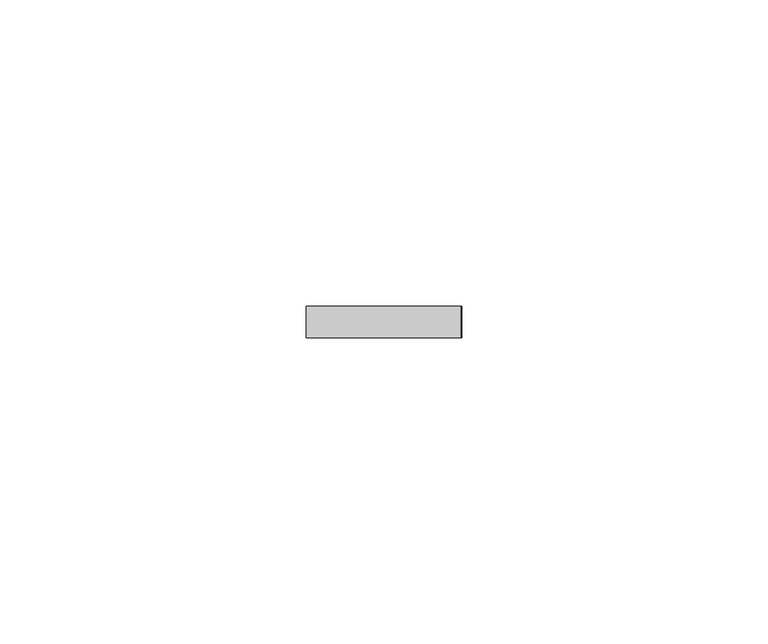
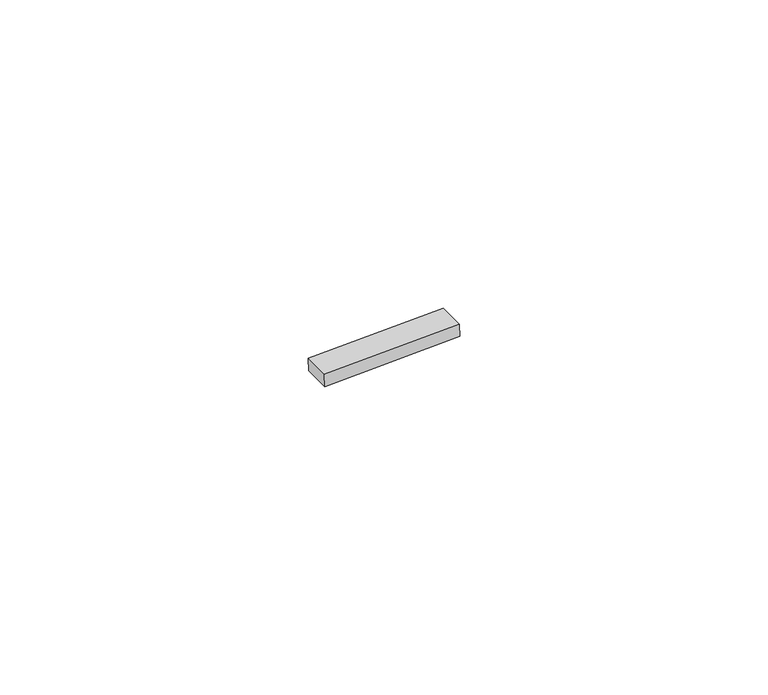
"""IFC4 building model written with IfcOpenShell, lengths in millimetres: proxy geometry, Inner panel:Inner panel:1:Inner panel:1 : Inner panel:Inner panel:300324:2:Inner panel:1:Inner panel:1 : Inner panel:Inner panel:300324:2 : Inner panel:Inner panel:1:Inner panel:1 : Inner panel:Inner panel:300324:300043:149 : Inner panel:Inner panel:1:Inner panel:1 : Inner panel:Inner panel:300324:2:Inner panel:1:Inner panel:1 : Inner panel:Inner panel:300324:2 : Inner panel:Inner panel:1:Inner panel:1 : Inner panel:Inner panel:300324:300043:308120."""

from ifc_helpers import new_model, si_unit, frame, origin, place, context, project, spatial, polyline, outline, extrude, source, transform, mapped, element, save


def generic_models_3277445f(model_context):
    return source(origin(), model_context, "Body", "SweptSolid", [
        extrude(outline(polyline([(0.0, -25.3999999), (0.0, 0.0), (5.2138089, 0.0), (5.2138089, -25.3999999), (0.0, -25.3999999)])), frame((558296.2989334, -578534.9848948, 3863.6749017), z_axis=(-0.041630544712223896, 0.0, 0.9991330730923502), x_axis=(0.0, -1.0, 0.0)), (0.0, 0.0, 1.0), 2.4763745),
    ])


if __name__ == "__main__":
    model = new_model("IFC4")
    model_context = context("Model", 3, world=origin())
    ifc_project = project(units=[si_unit("LENGTHUNIT", "METRE", prefix="MILLI")], contexts=[model_context])
    site = spatial("IfcSite", under=ifc_project)
    building = spatial("IfcBuilding", under=site)
    placement = place(None, origin())
    generic_models_shape = generic_models_3277445f(model_context)
    element("IfcBuildingElementProxy", 1, Name="Inner panel:Inner panel:1:Inner panel:1 : Inner panel:Inner panel:300324:2:Inner panel:1:Inner panel:1 : Inner panel:Inner panel:300324:2 : Inner panel:Inner panel:1:Inner panel:1 : Inner panel:Inner panel:300324:300043:149 : Inner panel:Inner panel:1:Inner panel:1 : Inner panel:Inner panel:300324:2:Inner panel:1:Inner panel:1 : Inner panel:Inner panel:300324:2 : Inner panel:Inner panel:1:Inner panel:1 : Inner panel:Inner panel:300324:300043:308120", ObjectType="Inner panel:Inner panel:1:Inner panel:1 : Inner panel:Inner panel:300324:2:Inner panel:1:Inner panel:1 : Inner panel:Inner panel:300324:2 : Inner panel:Inner panel:1:Inner panel:1 : Inner panel:Inner panel:300324:300043:149 : Inner panel:Inner panel:1:Inner panel:1 : Inner panel:Inner panel:300324:2:Inner panel:1:Inner panel:1 : Inner panel:Inner panel:300324:2 : Inner panel:Inner panel:1:Inner panel:1 : Inner panel:Inner panel:300324:300043:308120", at=placement, inside=building, context=model_context, shape_type="MappedRepresentation", body=[
        mapped(generic_models_shape, transform((0.0, 0.0, 0.0), x_axis=(1.0, 0.0, 0.0), y_axis=(0.0, 1.0, 0.0), z_axis=(0.0, 0.0, 1.0))),
    ])
    save(model, "model.ifc")

# Revit data of these elements
# Type "Inner panel:Inner panel:1:Inner panel:1 : Inner panel:Inner panel:300324:2:Inner panel:1:Inner panel:1 : Inner panel:Inner panel:300324:2 : Inner panel:Inner panel:1:Inner panel:1 : Inner panel:Inner panel:300324:300043:149 : Inner panel:Inner panel:1:Inner panel:1 : Inner panel:Inner panel:300324:2:Inner panel:1:Inner panel:1 : Inner panel:Inner panel:300324:2 : Inner panel:Inner panel:1:Inner panel:1 : Inner panel:Inner panel:300324:300043:308120"
#   NameOverride = "Inner panel:Inner panel:1:Inner panel:1 : Inner panel:Inner panel:300324:2:Inner panel:1:Inner panel:1 : Inner panel:Inner panel:300324:2 : Inner panel:Inner panel:1:Inner panel:1 : Inner panel:Inner panel:300324:300043:308120"
#   ObjectTypeOverride = "Inner panel:1:Inner panel:1 : Inner panel:Inner panel:300324:2 : Inner panel:Inner panel:1:Inner panel:1 : Inner panel:Inner panel:300324:300043"
#   Reference = "Inner panel"
#   Tag = "308120"
# Element 1 (IfcBuildingElementProxy, "Inner panel:Inner panel:1:Inner panel:1 : Inner panel:Inner panel:300324:2:Inner panel:1:Inner panel:1 : Inner panel:Inner panel:300324:2 : Inner panel:Inner panel:1:Inner panel:1 : Inner panel:Inner panel:300324:300043:149 : Inner panel:Inner panel:1:Inner panel:1 : Inner panel:Inner panel:300324:2:Inner panel:1:Inner panel:1 : Inner panel:Inner panel:300324:2 : Inner panel:Inner panel:1:Inner panel:1 : Inner panel:Inner panel:300324:300043:308120")
#   Materials on its faces: "AT CLIP - 1\" WIDE NON ABSORBENT, WEATHER-RESISTANT NEOPRENE/EPDM/SBR FOAM"
# Materials
#   "AT CLIP - 1\" WIDE NON ABSORBENT, WEATHER-RESISTANT NEOPRENE/EPDM/SBR FOAM": class "Generic", colour RGB 85 85 85, transparency 0, Cost = 0
